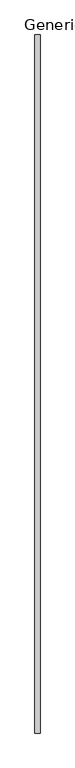
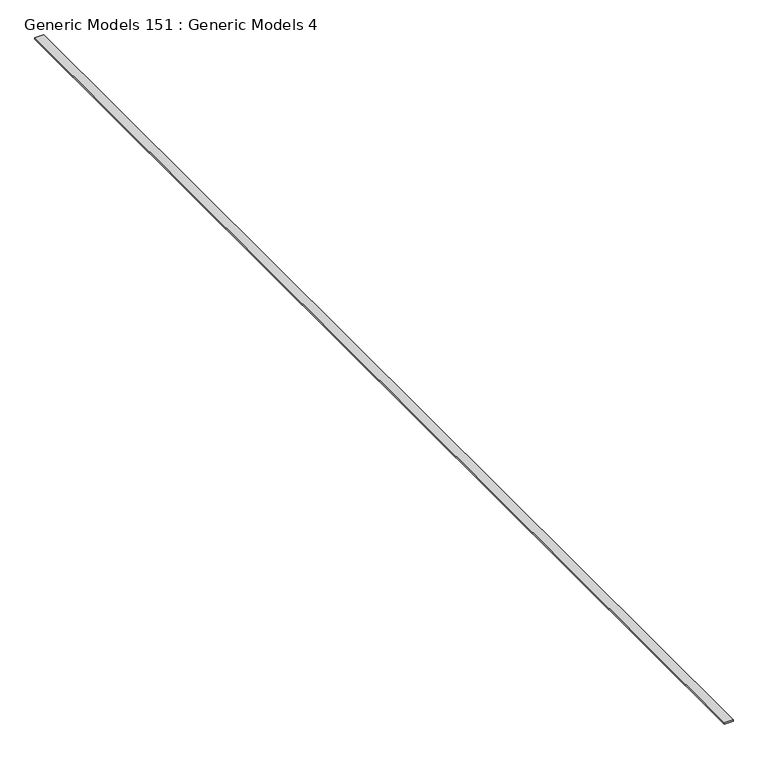
"""IFC4 building model written with IfcOpenShell, lengths in millimetres: proxy geometry, Generic Models 151 : Generic Models 4."""

import ifcopenshell
import ifcopenshell.guid

model = None  # the IFC model being written
_history = None  # IfcOwnerHistory: only IFC2X3 demands one
_inside = {}  # id of a spatial element -> (the spatial element, [elements in it])
_under = {}  # id of a project, library or spatial element -> (it, [spatial elements below it])
_declared = {}  # id of a project -> (the project, [libraries it declares])
_typed = {}  # id of a type object -> (the type object, [elements of that type])
_made_of = {}  # id of a material, layer set ... -> (it, [elements and type objects made of it])


def new_model(schema):
    """Start an empty IFC model of exactly this schema.

    Asked for "IFC4X3", IfcOpenShell would pick the latest addendum, in which some entities
    have other attributes; the version numbers below select the first issue.
    IFC2X3 requires an IfcOwnerHistory on every rooted entity: one is made here for all.
    """
    global model, _history
    if schema == "IFC4X3":
        model = ifcopenshell.file(schema_version=(4, 3, 0, 0))
    else:
        model = ifcopenshell.file(schema=schema)
    _inside.clear()
    _under.clear()
    _declared.clear()
    _typed.clear()
    _made_of.clear()
    _history = None
    if model.schema == "IFC2X3":
        org = make("IfcOrganization", Name="unknown")
        user = make(
            "IfcPersonAndOrganization",
            ThePerson=make("IfcPerson", FamilyName="unknown"),
            TheOrganization=org,
        )
        app = make(
            "IfcApplication",
            ApplicationDeveloper=org,
            Version="unknown",
            ApplicationFullName="unknown",
            ApplicationIdentifier="unknown",
        )
        _history = make(
            "IfcOwnerHistory",
            OwningUser=user,
            OwningApplication=app,
            ChangeAction="ADDED",
            CreationDate=0,
        )
    return model


def make(cls, **values):
    """One entity of the class cls with the attributes given. An attribute that is None is left unset."""
    return model.create_entity(
        cls, **{name: value for name, value in values.items() if value is not None}
    )


def rooted(cls, **values):
    """An entity with a GlobalId (a new one), such as an element, a storey or a relation."""
    return make(cls, GlobalId=ifcopenshell.guid.new(), OwnerHistory=_history, **values)


def si_unit(unit_type, name, prefix=None):
    """IfcSIUnit, for example si_unit("LENGTHUNIT", "METRE", prefix="MILLI")."""
    return make("IfcSIUnit", UnitType=unit_type, Prefix=prefix, Name=name)


def assignment(units):
    """IfcUnitAssignment: the units of a project."""
    return None if units is None else make("IfcUnitAssignment", Units=units)


def point(xyz):
    """IfcCartesianPoint."""
    return None if xyz is None else make("IfcCartesianPoint", Coordinates=xyz)


def direction(xyz):
    """IfcDirection."""
    return None if xyz is None else make("IfcDirection", DirectionRatios=xyz)


def frame(location, z_axis=None, x_axis=None):
    """IfcAxis2Placement3D, a coordinate frame: its origin and axes. An axis left out is left unset."""
    return make(
        "IfcAxis2Placement3D",
        Location=point(location),
        Axis=direction(z_axis),
        RefDirection=direction(x_axis),
    )


def origin():
    """The frame at (0, 0, 0) with its axes left unset."""
    return frame((0.0, 0.0, 0.0))


def place(relative_to, where):
    """IfcLocalPlacement: puts the frame where relative to a parent placement (None: the world)."""
    return make(
        "IfcLocalPlacement", PlacementRelTo=relative_to, RelativePlacement=where
    )


def context(
    kind, dimensions, precision=None, world=None, true_north=None, identifier=None
):
    """IfcGeometricRepresentationContext, for example the 3D "Model" context."""
    return make(
        "IfcGeometricRepresentationContext",
        ContextIdentifier=identifier,
        ContextType=kind,
        CoordinateSpaceDimension=dimensions,
        Precision=precision,
        WorldCoordinateSystem=world,
        TrueNorth=true_north,
    )


def project(units=None, contexts=None):
    """IfcProject with its units and contexts."""
    return rooted(
        "IfcProject",
        Name="project",
        RepresentationContexts=contexts,
        UnitsInContext=assignment(units),
    )


def spatial(cls, under=None, at=None, **own):
    """A site, building, storey or space (cls), placed at a placement, below another one or the project."""
    s = rooted(cls, ObjectPlacement=at, **own)
    if under is not None:
        _under.setdefault(under.id(), (under, []))[1].append(s)
    return s


def polyline(points):
    """IfcPolyline through the points."""
    return make("IfcPolyline", Points=[point(p) for p in points])


def outline(outer, holes=None, kind="AREA"):
    """IfcArbitraryClosedProfileDef: a profile drawn as a closed curve; with holes, ...WithVoids."""
    if holes is None:
        return make("IfcArbitraryClosedProfileDef", ProfileType=kind, OuterCurve=outer)
    return make(
        "IfcArbitraryProfileDefWithVoids",
        ProfileType=kind,
        OuterCurve=outer,
        InnerCurves=holes,
    )


def extrude(swept, where, along, depth):
    """IfcExtrudedAreaSolid: the profile swept, set in the frame where, extruded along a direction by depth."""
    return make(
        "IfcExtrudedAreaSolid",
        SweptArea=swept,
        Position=where,
        ExtrudedDirection=direction(along),
        Depth=depth,
    )


def shape(context_of_items, identifier, shape_type, items):
    """IfcShapeRepresentation: the items that make up one representation, for example the "Body"."""
    return make(
        "IfcShapeRepresentation",
        ContextOfItems=context_of_items,
        RepresentationIdentifier=identifier,
        RepresentationType=shape_type,
        Items=items,
    )


def source(mapping_origin, context_of_items, identifier, shape_type, items):
    """IfcRepresentationMap: a shape defined once, which mapped items show again and again."""
    return make(
        "IfcRepresentationMap",
        MappingOrigin=mapping_origin,
        MappedRepresentation=shape(context_of_items, identifier, shape_type, items),
    )


def transform(
    local_origin,
    x_axis=None,
    y_axis=None,
    z_axis=None,
    scale=None,
    scale2=None,
    scale3=None,
    uniform=True,
):
    """IfcCartesianTransformationOperator3D, or its non-uniform kind. x_axis, y_axis, z_axis: its Axis1, 2, 3."""
    if uniform:
        return make(
            "IfcCartesianTransformationOperator3D",
            Axis1=direction(x_axis),
            Axis2=direction(y_axis),
            LocalOrigin=point(local_origin),
            Scale=scale,
            Axis3=direction(z_axis),
        )
    return make(
        "IfcCartesianTransformationOperator3DnonUniform",
        Axis1=direction(x_axis),
        Axis2=direction(y_axis),
        LocalOrigin=point(local_origin),
        Scale=scale,
        Axis3=direction(z_axis),
        Scale2=scale2,
        Scale3=scale3,
    )


def mapped(mapping_source, mapping_target):
    """IfcMappedItem: shows the shape of a source again, moved by a transform."""
    return make(
        "IfcMappedItem", MappingSource=mapping_source, MappingTarget=mapping_target
    )


def made_of(thing, what):
    """Note that an element or type object is made of a material, layer set ...; save() writes the relation."""
    if what is not None:
        _made_of.setdefault(what.id(), (what, []))[1].append(thing)
    return thing


def element(
    cls,
    number,
    at=None,
    inside=None,
    cuts=None,
    type_object=None,
    material=None,
    context=None,
    identifier="Body",
    shape_type=None,
    held_by="IfcProductDefinitionShape",
    body=None,
    shapes=None,
    **own,
):
    """One element of the class cls, such as IfcWall. Its Tag is "e" and its number.

    at: its placement. inside: the storey or other place that contains it. cuts: it is an
    opening in that element (IfcRelVoidsElement). A single representation is given by context,
    identifier, shape_type and body (its items); several are given by shapes. held_by: the class
    of the entity that holds the representations. save() writes the other relations.
    """
    e = rooted(cls, Tag="e%d" % number, ObjectPlacement=at, **own)
    if body is not None:
        shapes = [shape(context, identifier, shape_type, body)]
    if shapes is not None:
        e.Representation = make(held_by, Representations=shapes)
    if inside is not None:
        _inside.setdefault(inside.id(), (inside, []))[1].append(e)
    if cuts is not None:
        rooted(
            "IfcRelVoidsElement", RelatingBuildingElement=cuts, RelatedOpeningElement=e
        )
    if type_object is not None:
        _typed.setdefault(type_object.id(), (type_object, []))[1].append(e)
    return made_of(e, material)


def aggregate(whole, parts):
    """IfcRelAggregates: a whole, such as a stair, and the parts it consists of."""
    return rooted("IfcRelAggregates", RelatingObject=whole, RelatedObjects=parts)


def save(model, path):
    """Write the relations noted so far, then the file.

    IfcRelAggregates (storeys below a building ...), IfcRelContainedInSpatialStructure (elements
    in a storey), IfcRelDefinesByType, IfcRelAssociatesMaterial and IfcRelDeclares: one each for
    every whole, place, type object, material and project.
    """
    for whole, parts in _under.values():
        aggregate(whole, parts)
    for where, things in _inside.values():
        rooted(
            "IfcRelContainedInSpatialStructure",
            RelatedElements=things,
            RelatingStructure=where,
        )
    for kind, things in _typed.values():
        rooted("IfcRelDefinesByType", RelatedObjects=things, RelatingType=kind)
    for what, things in _made_of.values():
        rooted("IfcRelAssociatesMaterial", RelatedObjects=things, RelatingMaterial=what)
    for by, libraries in _declared.values():
        rooted("IfcRelDeclares", RelatingContext=by, RelatedDefinitions=libraries)
    model.write(path)


def generic_models_151_generic_models_4_3005bbfc(model_context):
    return source(origin(), model_context, "Body", "SweptSolid", [
        extrude(outline(polyline([(-6508.088527, -6864.9230338), (-6610.5236296, -6864.9230338), (-6610.5236296, 7054.2769662), (-6508.088527, 7054.2769662), (-6508.088527, -6864.9230338)])), frame((0.0, 0.0, 126194.3578287), z_axis=(0.0, 0.0, 1.0), x_axis=(1.0, 0.0, 0.0)), (0.0, 0.0, 1.0), 17.0499747),
    ])


if __name__ == "__main__":
    model = new_model("IFC4")
    model_context = context("Model", 3, world=origin())
    ifc_project = project(units=[si_unit("LENGTHUNIT", "METRE", prefix="MILLI")], contexts=[model_context])
    site = spatial("IfcSite", under=ifc_project)
    building = spatial("IfcBuilding", under=site)
    placement = place(None, origin())
    generic_models_151_generic_models_4_shape = generic_models_151_generic_models_4_3005bbfc(model_context)
    element("IfcBuildingElementProxy", 1, Name="Generic Models 151 : Generic Models 4", ObjectType="Generic Models 151 : Generic Models 4", at=placement, inside=building, context=model_context, shape_type="MappedRepresentation", body=[
        mapped(generic_models_151_generic_models_4_shape, transform((0.0, 0.0, 0.0), x_axis=(1.0, 0.0, 0.0), y_axis=(0.0, 1.0, 0.0), z_axis=(0.0, 0.0, 1.0))),
    ])
    save(model, "model.ifc")

# Revit data of these elements
# Element 1 (IfcBuildingElementProxy, "Generic Models 151 : Generic Models 4")
#   Materials on its faces: "_2X BLOCKING AS REQUIRED"
# Materials
#   "_2X BLOCKING AS REQUIRED": class "Generic", colour RGB 177 130 114, transparency 0, Cost = 0
